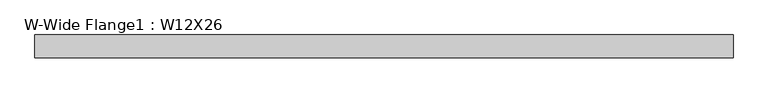
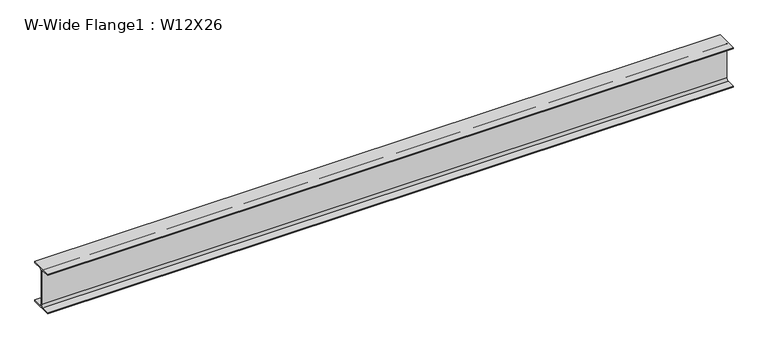
"""IFC4 building model written with IfcOpenShell, lengths in millimetres: beam geometry, W-Wide Flange1 : W12X26."""

import ifcopenshell
import ifcopenshell.guid

model = None  # the IFC model being written
_history = None  # IfcOwnerHistory: only IFC2X3 demands one
_inside = {}  # id of a spatial element -> (the spatial element, [elements in it])
_under = {}  # id of a project, library or spatial element -> (it, [spatial elements below it])
_declared = {}  # id of a project -> (the project, [libraries it declares])
_typed = {}  # id of a type object -> (the type object, [elements of that type])
_made_of = {}  # id of a material, layer set ... -> (it, [elements and type objects made of it])


def new_model(schema):
    """Start an empty IFC model of exactly this schema.

    Asked for "IFC4X3", IfcOpenShell would pick the latest addendum, in which some entities
    have other attributes; the version numbers below select the first issue.
    IFC2X3 requires an IfcOwnerHistory on every rooted entity: one is made here for all.
    """
    global model, _history
    if schema == "IFC4X3":
        model = ifcopenshell.file(schema_version=(4, 3, 0, 0))
    else:
        model = ifcopenshell.file(schema=schema)
    _inside.clear()
    _under.clear()
    _declared.clear()
    _typed.clear()
    _made_of.clear()
    _history = None
    if model.schema == "IFC2X3":
        org = make("IfcOrganization", Name="unknown")
        user = make(
            "IfcPersonAndOrganization",
            ThePerson=make("IfcPerson", FamilyName="unknown"),
            TheOrganization=org,
        )
        app = make(
            "IfcApplication",
            ApplicationDeveloper=org,
            Version="unknown",
            ApplicationFullName="unknown",
            ApplicationIdentifier="unknown",
        )
        _history = make(
            "IfcOwnerHistory",
            OwningUser=user,
            OwningApplication=app,
            ChangeAction="ADDED",
            CreationDate=0,
        )
    return model


def make(cls, **values):
    """One entity of the class cls with the attributes given. An attribute that is None is left unset."""
    return model.create_entity(
        cls, **{name: value for name, value in values.items() if value is not None}
    )


def rooted(cls, **values):
    """An entity with a GlobalId (a new one), such as an element, a storey or a relation."""
    return make(cls, GlobalId=ifcopenshell.guid.new(), OwnerHistory=_history, **values)


def si_unit(unit_type, name, prefix=None):
    """IfcSIUnit, for example si_unit("LENGTHUNIT", "METRE", prefix="MILLI")."""
    return make("IfcSIUnit", UnitType=unit_type, Prefix=prefix, Name=name)


def assignment(units):
    """IfcUnitAssignment: the units of a project."""
    return None if units is None else make("IfcUnitAssignment", Units=units)


def point(xyz):
    """IfcCartesianPoint."""
    return None if xyz is None else make("IfcCartesianPoint", Coordinates=xyz)


def direction(xyz):
    """IfcDirection."""
    return None if xyz is None else make("IfcDirection", DirectionRatios=xyz)


def frame(location, z_axis=None, x_axis=None):
    """IfcAxis2Placement3D, a coordinate frame: its origin and axes. An axis left out is left unset."""
    return make(
        "IfcAxis2Placement3D",
        Location=point(location),
        Axis=direction(z_axis),
        RefDirection=direction(x_axis),
    )


def frame_2d(location, x_axis=None):
    """IfcAxis2Placement2D, a coordinate frame in the plane: its origin and x axis."""
    return make(
        "IfcAxis2Placement2D", Location=point(location), RefDirection=direction(x_axis)
    )


def origin():
    """The frame at (0, 0, 0) with its axes left unset."""
    return frame((0.0, 0.0, 0.0))


def place(relative_to, where):
    """IfcLocalPlacement: puts the frame where relative to a parent placement (None: the world)."""
    return make(
        "IfcLocalPlacement", PlacementRelTo=relative_to, RelativePlacement=where
    )


def context(
    kind, dimensions, precision=None, world=None, true_north=None, identifier=None
):
    """IfcGeometricRepresentationContext, for example the 3D "Model" context."""
    return make(
        "IfcGeometricRepresentationContext",
        ContextIdentifier=identifier,
        ContextType=kind,
        CoordinateSpaceDimension=dimensions,
        Precision=precision,
        WorldCoordinateSystem=world,
        TrueNorth=true_north,
    )


def project(units=None, contexts=None):
    """IfcProject with its units and contexts."""
    return rooted(
        "IfcProject",
        Name="project",
        RepresentationContexts=contexts,
        UnitsInContext=assignment(units),
    )


def spatial(cls, under=None, at=None, **own):
    """A site, building, storey or space (cls), placed at a placement, below another one or the project."""
    s = rooted(cls, ObjectPlacement=at, **own)
    if under is not None:
        _under.setdefault(under.id(), (under, []))[1].append(s)
    return s


def polyline(points):
    """IfcPolyline through the points."""
    return make("IfcPolyline", Points=[point(p) for p in points])


def circle_curve(where, radius):
    """IfcCircle in the frame where."""
    return make("IfcCircle", Position=where, Radius=radius)


def trimmed(basis, trim1, trim2, sense, master):
    """IfcTrimmedCurve: the piece of a basis curve between two trims."""
    return make(
        "IfcTrimmedCurve",
        BasisCurve=basis,
        Trim1=trim1,
        Trim2=trim2,
        SenseAgreement=sense,
        MasterRepresentation=master,
    )


def segment(curve, same_sense, transition):
    """IfcCompositeCurveSegment."""
    return make(
        "IfcCompositeCurveSegment",
        Transition=transition,
        SameSense=same_sense,
        ParentCurve=curve,
    )


def composite_curve(segments, self_intersect=None):
    """IfcCompositeCurve: segments joined end to end."""
    return make("IfcCompositeCurve", Segments=segments, SelfIntersect=self_intersect)


def outline(outer, holes=None, kind="AREA"):
    """IfcArbitraryClosedProfileDef: a profile drawn as a closed curve; with holes, ...WithVoids."""
    if holes is None:
        return make("IfcArbitraryClosedProfileDef", ProfileType=kind, OuterCurve=outer)
    return make(
        "IfcArbitraryProfileDefWithVoids",
        ProfileType=kind,
        OuterCurve=outer,
        InnerCurves=holes,
    )


def extrude(swept, where, along, depth):
    """IfcExtrudedAreaSolid: the profile swept, set in the frame where, extruded along a direction by depth."""
    return make(
        "IfcExtrudedAreaSolid",
        SweptArea=swept,
        Position=where,
        ExtrudedDirection=direction(along),
        Depth=depth,
    )


def shape(context_of_items, identifier, shape_type, items):
    """IfcShapeRepresentation: the items that make up one representation, for example the "Body"."""
    return make(
        "IfcShapeRepresentation",
        ContextOfItems=context_of_items,
        RepresentationIdentifier=identifier,
        RepresentationType=shape_type,
        Items=items,
    )


def source(mapping_origin, context_of_items, identifier, shape_type, items):
    """IfcRepresentationMap: a shape defined once, which mapped items show again and again."""
    return make(
        "IfcRepresentationMap",
        MappingOrigin=mapping_origin,
        MappedRepresentation=shape(context_of_items, identifier, shape_type, items),
    )


def transform(
    local_origin,
    x_axis=None,
    y_axis=None,
    z_axis=None,
    scale=None,
    scale2=None,
    scale3=None,
    uniform=True,
):
    """IfcCartesianTransformationOperator3D, or its non-uniform kind. x_axis, y_axis, z_axis: its Axis1, 2, 3."""
    if uniform:
        return make(
            "IfcCartesianTransformationOperator3D",
            Axis1=direction(x_axis),
            Axis2=direction(y_axis),
            LocalOrigin=point(local_origin),
            Scale=scale,
            Axis3=direction(z_axis),
        )
    return make(
        "IfcCartesianTransformationOperator3DnonUniform",
        Axis1=direction(x_axis),
        Axis2=direction(y_axis),
        LocalOrigin=point(local_origin),
        Scale=scale,
        Axis3=direction(z_axis),
        Scale2=scale2,
        Scale3=scale3,
    )


def mapped(mapping_source, mapping_target):
    """IfcMappedItem: shows the shape of a source again, moved by a transform."""
    return make(
        "IfcMappedItem", MappingSource=mapping_source, MappingTarget=mapping_target
    )


def made_of(thing, what):
    """Note that an element or type object is made of a material, layer set ...; save() writes the relation."""
    if what is not None:
        _made_of.setdefault(what.id(), (what, []))[1].append(thing)
    return thing


def element(
    cls,
    number,
    at=None,
    inside=None,
    cuts=None,
    type_object=None,
    material=None,
    context=None,
    identifier="Body",
    shape_type=None,
    held_by="IfcProductDefinitionShape",
    body=None,
    shapes=None,
    **own,
):
    """One element of the class cls, such as IfcWall. Its Tag is "e" and its number.

    at: its placement. inside: the storey or other place that contains it. cuts: it is an
    opening in that element (IfcRelVoidsElement). A single representation is given by context,
    identifier, shape_type and body (its items); several are given by shapes. held_by: the class
    of the entity that holds the representations. save() writes the other relations.
    """
    e = rooted(cls, Tag="e%d" % number, ObjectPlacement=at, **own)
    if body is not None:
        shapes = [shape(context, identifier, shape_type, body)]
    if shapes is not None:
        e.Representation = make(held_by, Representations=shapes)
    if inside is not None:
        _inside.setdefault(inside.id(), (inside, []))[1].append(e)
    if cuts is not None:
        rooted(
            "IfcRelVoidsElement", RelatingBuildingElement=cuts, RelatedOpeningElement=e
        )
    if type_object is not None:
        _typed.setdefault(type_object.id(), (type_object, []))[1].append(e)
    return made_of(e, material)


def aggregate(whole, parts):
    """IfcRelAggregates: a whole, such as a stair, and the parts it consists of."""
    return rooted("IfcRelAggregates", RelatingObject=whole, RelatedObjects=parts)


def save(model, path):
    """Write the relations noted so far, then the file.

    IfcRelAggregates (storeys below a building ...), IfcRelContainedInSpatialStructure (elements
    in a storey), IfcRelDefinesByType, IfcRelAssociatesMaterial and IfcRelDeclares: one each for
    every whole, place, type object, material and project.
    """
    for whole, parts in _under.values():
        aggregate(whole, parts)
    for where, things in _inside.values():
        rooted(
            "IfcRelContainedInSpatialStructure",
            RelatedElements=things,
            RelatingStructure=where,
        )
    for kind, things in _typed.values():
        rooted("IfcRelDefinesByType", RelatedObjects=things, RelatingType=kind)
    for what, things in _made_of.values():
        rooted("IfcRelAssociatesMaterial", RelatedObjects=things, RelatingMaterial=what)
    for by, libraries in _declared.values():
        rooted("IfcRelDeclares", RelatingContext=by, RelatedDefinitions=libraries)
    model.write(path)


def w_wide_flange1_w12x26_7ef256fb(model_context):
    return source(origin(), model_context, "Body", "SweptSolid", [
        extrude(outline(composite_curve([segment(polyline([(82.423, -145.288), (82.423, -154.94), (-82.423, -154.94), (-82.423, -145.288), (-20.2565, -145.288)]), True, "CONTINUOUS"), segment(trimmed(circle_curve(frame_2d((-20.2565, -127.9525)), 17.3355), [point((-20.2565, -145.288))], [point((-2.921, -127.9525))], True, "CARTESIAN"), True, "CONTINUOUS"), segment(polyline([(-2.921, -127.9525), (-2.921, 127.9525)]), True, "CONTINUOUS"), segment(trimmed(circle_curve(frame_2d((-20.2565, 127.9525)), 17.3355), [point((-2.921, 127.9525))], [point((-20.2565, 145.288))], True, "CARTESIAN"), True, "CONTINUOUS"), segment(polyline([(-20.2565, 145.288), (-82.423, 145.288), (-82.423, 154.94), (82.423, 154.94), (82.423, 145.288), (20.2565, 145.288)]), True, "CONTINUOUS"), segment(trimmed(circle_curve(frame_2d((20.2565, 127.9525)), 17.3355), [point((20.2565, 145.288))], [point((2.921, 127.9525))], True, "CARTESIAN"), True, "CONTINUOUS"), segment(polyline([(2.921, 127.9525), (2.921, -127.9525)]), True, "CONTINUOUS"), segment(trimmed(circle_curve(frame_2d((20.2565, -127.9525)), 17.3355), [point((2.921, -127.9525))], [point((20.2565, -145.288))], True, "CARTESIAN"), True, "CONTINUOUS"), segment(polyline([(20.2565, -145.288), (82.423, -145.288)]), True, "CONTINUOUS")], self_intersect=False)), frame((-2476.8883988, 0.0, 0.0), z_axis=(1.0, 0.0, 0.0), x_axis=(0.0, 1.0, 0.0)), (0.0, 0.0, 1.0), 5054.9957976),
    ])


if __name__ == "__main__":
    model = new_model("IFC4")
    model_context = context("Model", 3, world=origin())
    ifc_project = project(units=[si_unit("LENGTHUNIT", "METRE", prefix="MILLI")], contexts=[model_context])
    site = spatial("IfcSite", under=ifc_project)
    building = spatial("IfcBuilding", under=site)
    placement = place(None, origin())
    w_wide_flange1_w12x26_shape = w_wide_flange1_w12x26_7ef256fb(model_context)
    element("IfcBeam", 1, ObjectType="W-Wide Flange1 : W12X26", at=placement, inside=building, context=model_context, shape_type="MappedRepresentation", body=[
        mapped(w_wide_flange1_w12x26_shape, transform((0.0, 0.0, 0.0), x_axis=(1.0, 0.0, 0.0), y_axis=(0.0, 1.0, 0.0), z_axis=(0.0, 0.0, 1.0))),
    ])
    save(model, "model.ifc")

# Revit data of these elements
# Type "W-Wide Flange1 : W12X26"
#   Assembly Code = "B10"
#   W = 26
#   Start Extension Calculation [instance default] = 10' - 0"
#   Start Extension [instance default] = -0' - 0 1/2"
#   End Extension Calculation [instance default] = 10' - 0"
#   End Extension [instance default] = -0' - 0 1/2"
#   Length [instance default] = 5' - 0"
#   bf = 0' - 6.49"
#   d = 1' - 0.2"
#   k = 0' - 1 1/16"
#   k2 = 0' - 0.6825"
#   tf = 0' - 0.38"
#   tw = 0' - 0.23"
#   A = 0.053125 SF
#   Structural Material [instance default] = Metal - Steel - ASTM A992
# Element 1 (IfcBeam, "W-Wide Flange1 : W12X26")
#   Materials on its faces: "Metal - Steel - ASTM A992"
# Materials
#   "Metal - Steel - ASTM A992": class "Metal", colour RGB 199 199 199, transparency 0
